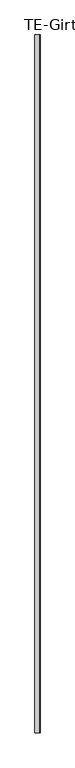
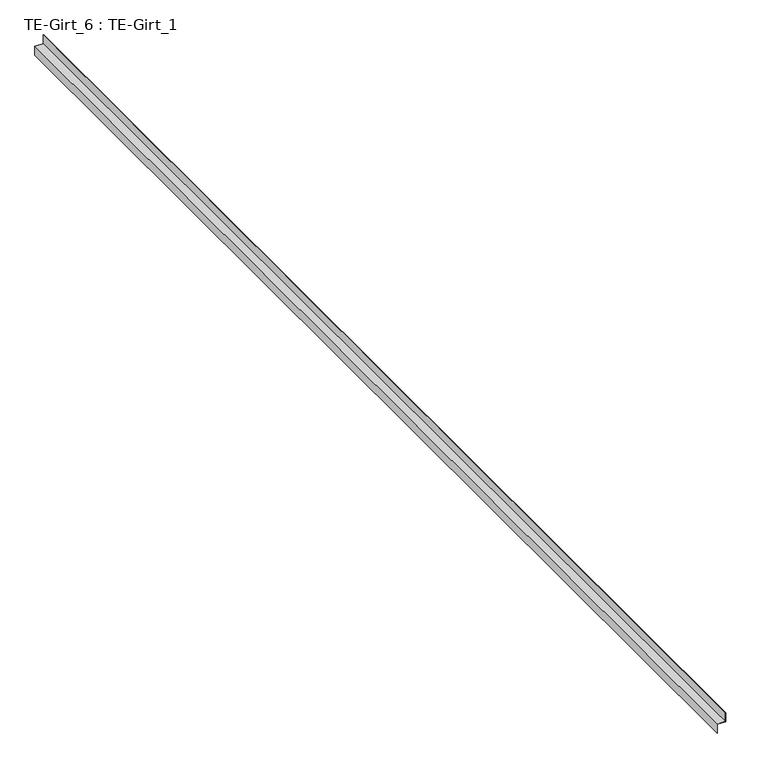
"""IFC4 building model written with IfcOpenShell, lengths in millimetres: proxy geometry, TE-Girt_6 : TE-Girt_1."""

from ifc_helpers import new_model, si_unit, frame, origin, place, context, project, spatial, polyline, outline, extrude, source, transform, mapped, element, save


def te_girt_6_te_girt_1_6a4ee48b(model_context):
    return source(origin(), model_context, "Body", "SweptSolid", [
        extrude(outline(polyline([(2374.9, 590353.5827614), (2413.0, 590353.5827614), (2413.0, 590352.6897927), (2375.7929688, 590352.6897927), (2375.7929688, 590318.6434739), (2337.6929688, 590318.6434739), (2337.6929688, 590319.5364427), (2374.9, 590319.5364427), (2374.9, 590353.5827614)])), frame((0.0, -536417.5913841, 0.0), z_axis=(0.0, 1.0, 0.0), x_axis=(0.0, 0.0, 1.0)), (0.0, 0.0, 1.0), 4777.4820312),
    ])


if __name__ == "__main__":
    model = new_model("IFC4")
    model_context = context("Model", 3, world=origin())
    ifc_project = project(units=[si_unit("LENGTHUNIT", "METRE", prefix="MILLI")], contexts=[model_context])
    site = spatial("IfcSite", under=ifc_project)
    building = spatial("IfcBuilding", under=site)
    placement = place(None, origin())
    te_girt_6_te_girt_1_shape = te_girt_6_te_girt_1_6a4ee48b(model_context)
    element("IfcBuildingElementProxy", 1, Name="TE-Girt_6 : TE-Girt_1", ObjectType="TE-Girt_6 : TE-Girt_1", at=placement, inside=building, context=model_context, shape_type="MappedRepresentation", body=[
        mapped(te_girt_6_te_girt_1_shape, transform((0.0, 0.0, 0.0), x_axis=(1.0, 0.0, 0.0), y_axis=(0.0, 1.0, 0.0), z_axis=(0.0, 0.0, 1.0))),
    ])
    save(model, "model.ifc")

# Revit data of these elements
# Element 1 (IfcBuildingElementProxy, "TE-Girt_6 : TE-Girt_1")
#   Materials on its faces: "Z-FURRING, COLD-FORMED GALV."
# Materials
#   "Z-FURRING, COLD-FORMED GALV.": class "Generic", colour RGB 143 142 141, transparency 0, Cost = 0
